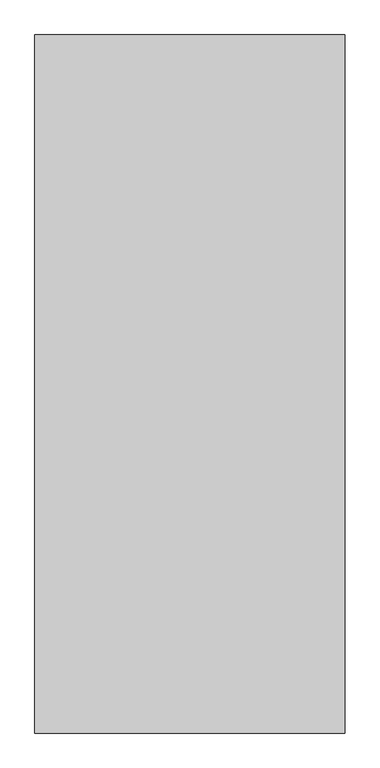
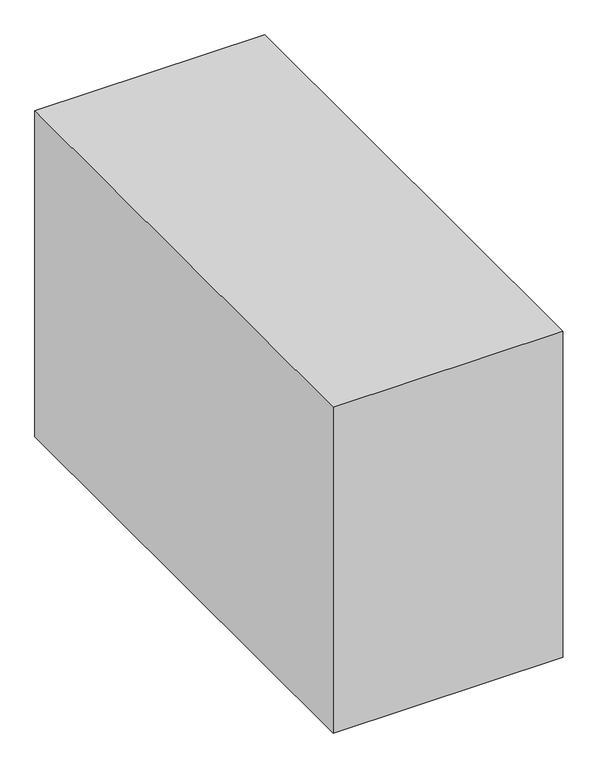
"""IFC4 building model written with IfcOpenShell, lengths in millimetres: proxy geometry, Space Planning Box_hec : Space Planning Box_hec."""

from ifc_helpers import new_model, si_unit, origin, origin_with_axes, place, context, project, spatial, polyline, outline, extrude, source, transform, mapped, element, save


def generic_models_29bcd6f9(model_context):
    return source(origin(), model_context, "Body", "SweptSolid", [
        extrude(outline(polyline([(2000.0, 4500.0), (2000.0, -4500.0), (-2000.0, -4500.0), (-2000.0, 4500.0), (2000.0, 4500.0)])), origin_with_axes(), (0.0, 0.0, 1.0), 6000.0),
    ])


if __name__ == "__main__":
    model = new_model("IFC4")
    model_context = context("Model", 3, world=origin())
    ifc_project = project(units=[si_unit("LENGTHUNIT", "METRE", prefix="MILLI")], contexts=[model_context])
    site = spatial("IfcSite", under=ifc_project)
    building = spatial("IfcBuilding", under=site)
    placement = place(None, origin())
    generic_models_shape = generic_models_29bcd6f9(model_context)
    element("IfcBuildingElementProxy", 1, Name="Space Planning Box_hec : Space Planning Box_hec", ObjectType="Space Planning Box_hec : Space Planning Box_hec", at=placement, inside=building, context=model_context, shape_type="MappedRepresentation", body=[
        mapped(generic_models_shape, transform((0.0, 0.0, 0.0), x_axis=(1.0, 0.0, 0.0), y_axis=(0.0, 1.0, 0.0), z_axis=(0.0, 0.0, 1.0))),
    ])
    save(model, "model.ifc")

# Revit data of these elements
# Type "Space Planning Box_hec : Space Planning Box_hec"
#   Type Comments = "..."
#   Room Name [instance default] = "?"
#   Interior Finish [instance default] = ""
#   Exterior Finish [instance default] = ""
#   Department [instance default] = ""
#   Assembly Code = "..."
#   Width [instance default] = 1524 mm
#   Program Area [instance default] = 0 m²
#   Length [instance default] = 1524 mm
#   Height [instance default] = 1524 mm
#   Area [instance default] = 2.32258 m²
#   Fill Color [instance default] = Cyan
#   Default Elevation = 0
# Element 1 (IfcBuildingElementProxy, "Space Planning Box_hec : Space Planning Box_hec")
#   Room Name = "Stairway"
#   Interior Finish = "IF2"
#   Exterior Finish = "EF1"
#   Department = "AR"
#   Width = 4000 mm
#   Program Area = 36 m²
#   Length = 9000 mm
#   Height = 6000 mm
#   Area = 36 m²
#   Fill Color = Lavender
#   Materials on its faces: "Lavender"
# Materials
#   "Cyan": class "Generic", colour RGB 0 255 255, transparency 0.2, Cost = 0
#   "Lavender": class "Generic", colour RGB 186 85 211, transparency 0.2, Cost = 0
